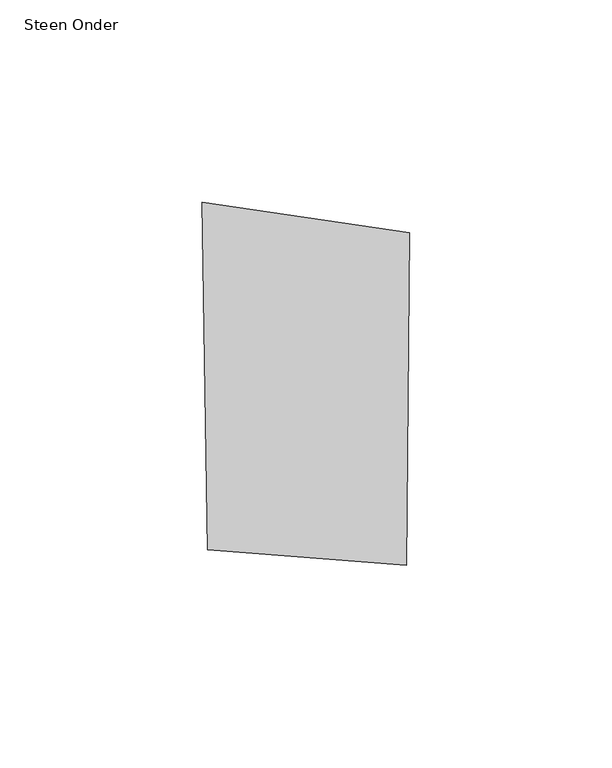
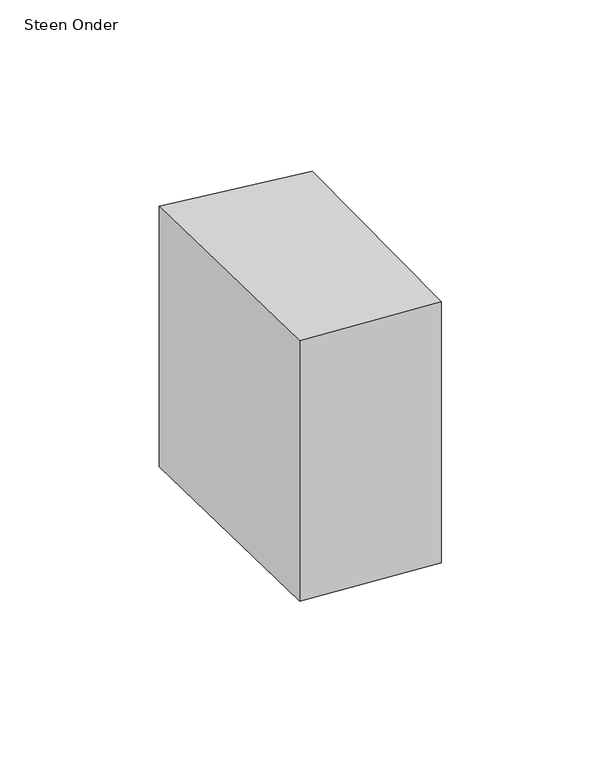
"""IFC4 building model written with IfcOpenShell, lengths in millimetres: proxy geometry, 00_GMA_steen_versie_4 : Steen Onder."""

from ifc_helpers import new_model, si_unit, origin, origin_with_axes, place, context, project, spatial, polyline, outline, extrude, source, transform, mapped, element, save


def steen_onder_0f4b40e1(model_context):
    return source(origin(), model_context, "Body", "SweptSolid", [
        extrude(outline(polyline([(100.9474258, 107.8911102), (100.2051758, 25.6709482), (51.0642407, 29.5523677), (49.7352921, 115.3315329), (100.9474258, 107.8911102)])), origin_with_axes(), (0.0, 0.0, 1.0), 100.0),
    ])


if __name__ == "__main__":
    model = new_model("IFC4")
    model_context = context("Model", 3, world=origin())
    ifc_project = project(units=[si_unit("LENGTHUNIT", "METRE", prefix="MILLI")], contexts=[model_context])
    site = spatial("IfcSite", under=ifc_project)
    building = spatial("IfcBuilding", under=site)
    placement = place(None, origin())
    steen_onder_shape = steen_onder_0f4b40e1(model_context)
    element("IfcBuildingElementProxy", 1, Name="00_GMA_steen_versie_4 : Steen Onder", ObjectType="00_GMA_steen_versie_4 : Steen Onder", at=placement, inside=building, context=model_context, shape_type="MappedRepresentation", body=[
        mapped(steen_onder_shape, transform((0.0, 0.0, 0.0), x_axis=(1.0, 0.0, 0.0), y_axis=(0.0, 1.0, 0.0), z_axis=(0.0, 0.0, 1.0))),
    ])
    save(model, "model.ifc")

# Revit data of these elements
# Type "00_GMA_steen_versie_4 : Steen Onder"
#   StootVoegHalfBoven [instance default] = 5 mm
#   StootVoegHalf [instance default] = 5 mm
#   StootVoegBreedteOnder = 10 mm
#   StootVoegBreedteBoven = 10 mm
#   Steendikte = 100 mm
#   LintVoegOnderHalf = 0 mm
#   LintVoegOnder = 0 mm
#   LintVoegBovenHalf = 5 mm
#   LintVoegBoven = 10 mm
#   materiaal = none
#   MateriaalVoeg = none
#   Default Elevation = 0
